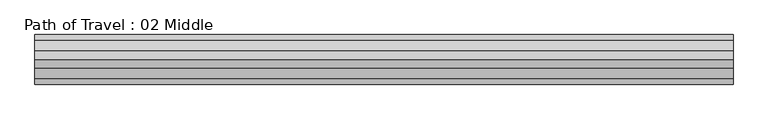
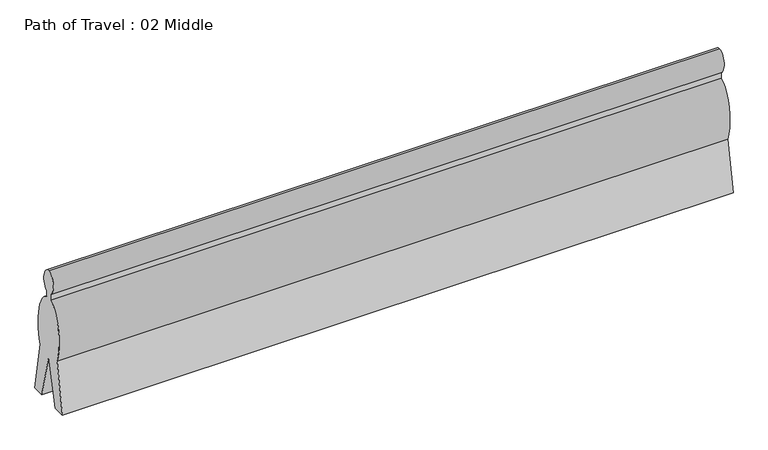
"""IFC4 building model written with IfcOpenShell, lengths in millimetres: proxy geometry, Path of Travel : 02 Middle."""

from ifc_helpers import new_model, si_unit, point, frame, origin, place, context, project, spatial, ellipse_curve, trimmed, source, transform, mapped, element, save
from ifc_brep_helpers import plane_surface, extruded_surface, advanced_brep


def path_of_travel_02_middle_f5177a39(model_context):
    return source(origin(), model_context, "Body", "AdvancedBrep", [
        advanced_brep(
        [(227.5554837, 0.0, 1727.2), (227.5554837, 42.9018657, 1436.6534209), (227.5554837, 42.9018657, 1363.4763406), (227.5554837, 184.1186263, 643.4144547), (227.5554837, 297.5699544, 0.0), (227.5554837, 145.6574193, 0.0), (227.5554837, 0.0, 584.2), (227.5554837, -145.6574193, 0.0), (227.5554837, -297.5699544, 0.0), (227.5554837, -184.1186263, 643.4144547), (227.5554837, -42.9018657, 1363.4763406), (227.5554837, -42.9018657, 1436.6534209), (8609.5554837, 0.0, 1727.2), (8609.5554837, -42.9018657, 1436.6534209), (8609.5554837, -42.9018657, 1363.4763406), (8609.5554837, -184.1186263, 643.4144547), (8609.5554837, -297.5699544, 0.0), (8609.5554837, -145.6574193, 0.0), (8609.5554837, 0.0, 584.2), (8609.5554837, 145.6574193, 0.0), (8609.5554837, 297.5699544, 0.0), (8609.5554837, 184.1186263, 643.4144547), (8609.5554837, 42.9018657, 1363.4763406), (8609.5554837, 42.9018657, 1436.6534209)],
        [
            (0, 1, ellipse_curve(frame((227.5554837, 0.0, 1574.8), z_axis=(-1.0, 0.0, 0.0), x_axis=(0.0, 0.0, 1.0)), 152.4, 101.6)),
            (1, 2),
            (2, 3, ellipse_curve(frame((227.5554837, 0.0, 914.4), z_axis=(-1.0, 0.0, 0.0), x_axis=(0.0, 0.0, -1.0)), 457.2, 228.6)),
            (3, 4),
            (4, 5),
            (5, 6),
            (6, 7),
            (7, 8),
            (8, 9),
            (9, 10, ellipse_curve(frame((227.5554837, 0.0, 914.4), z_axis=(-1.0, 0.0, 0.0), x_axis=(0.0, 0.0, -1.0)), 457.2, 228.6)),
            (10, 11),
            (11, 0, ellipse_curve(frame((227.5554837, 0.0, 1574.8), z_axis=(-1.0, 0.0, 0.0), x_axis=(0.0, 0.0, 1.0)), 152.4, 101.6)),
            (12, 13, ellipse_curve(frame((8609.5554837, 0.0, 1574.8), z_axis=(1.0, 0.0, 0.0), x_axis=(0.0, 0.0, 1.0)), 152.4, 101.6)),
            (13, 14),
            (14, 15, ellipse_curve(frame((8609.5554837, 0.0, 914.4), z_axis=(1.0, 0.0, 0.0), x_axis=(0.0, 0.0, -1.0)), 457.2, 228.6)),
            (15, 16),
            (16, 17),
            (17, 18),
            (18, 19),
            (19, 20),
            (20, 21),
            (21, 22, ellipse_curve(frame((8609.5554837, 0.0, 914.4), z_axis=(1.0, 0.0, 0.0), x_axis=(0.0, 0.0, -1.0)), 457.2, 228.6)),
            (22, 23),
            (23, 12, ellipse_curve(frame((8609.5554837, 0.0, 1574.8), z_axis=(1.0, 0.0, 0.0), x_axis=(0.0, 0.0, 1.0)), 152.4, 101.6)),
            (0, 12),
            (23, 1),
            (22, 2),
            (21, 3),
            (20, 4),
            (19, 5),
            (18, 6),
            (17, 7),
            (16, 8),
            (15, 9),
            (14, 10),
            (13, 11),
        ],
        [
            plane_surface(frame((227.5554837, 0.0, 0.0), z_axis=(-1.0, 0.0, 0.0), x_axis=(0.0, 0.0, 1.0))),
            plane_surface(frame((8609.5554837, 0.0, 0.0), z_axis=(1.0, 0.0, 0.0), x_axis=(0.0, 0.0, 1.0))),
            extruded_surface(trimmed(ellipse_curve(frame((8609.5554837, 0.0, 1574.8), z_axis=(-1.0, 0.0, 0.0), x_axis=(0.0, 0.0, 1.0)), 152.4, 101.6), [point((8609.5554837, 0.0, 1727.2))], [point((8609.5554837, 42.9018657, 1436.6534209))], True, "CARTESIAN"), (-8382.0, 0.0, 0.0), 8382.0),
            plane_surface(frame((227.5554837, 42.9018657, 1436.6534209), z_axis=(0.0, 1.0, 0.0), x_axis=(1.0, 0.0, 0.0))),
            extruded_surface(trimmed(ellipse_curve(frame((8609.5554837, 0.0, 914.4), z_axis=(-1.0, 0.0, 0.0), x_axis=(0.0, 0.0, -1.0)), 457.2, 228.6), [point((8609.5554837, 42.9018657, 1363.4763406))], [point((8609.5554837, 184.1186263, 643.4144547))], True, "CARTESIAN"), (-8382.0, 0.0, 0.0), 8382.0),
            plane_surface(frame((227.5554837, 184.1186263, 643.4144547), z_axis=(0.0, 0.9848077530122078, 0.17364817766693205), x_axis=(1.0, 0.0, 0.0))),
            plane_surface(frame((227.5554837, 297.5699544, 0.0), z_axis=(0.0, 0.0, -1.0), x_axis=(1.0, 0.0, 0.0))),
            plane_surface(frame((227.5554837, 145.6574193, 0.0), z_axis=(0.0, -0.9702957262760199, -0.2419218955995739), x_axis=(1.0, 0.0, 0.0))),
            plane_surface(frame((227.5554837, 0.0, 584.2), z_axis=(0.0, 0.9702957262759961, -0.24192189559966923), x_axis=(1.0, 0.0, 0.0))),
            plane_surface(frame((227.5554837, -145.6574193, 0.0), z_axis=(0.0, 0.0, -1.0), x_axis=(1.0, 0.0, 0.0))),
            plane_surface(frame((227.5554837, -297.5699544, 0.0), z_axis=(0.0, -0.984807753012208, 0.17364817766693066), x_axis=(1.0, 0.0, 0.0))),
            extruded_surface(trimmed(ellipse_curve(frame((8609.5554837, 0.0, 914.4), z_axis=(-1.0, 0.0, 0.0), x_axis=(0.0, 0.0, -1.0)), 457.2, 228.6), [point((8609.5554837, -184.1186263, 643.4144547))], [point((8609.5554837, -42.9018657, 1363.4763406))], True, "CARTESIAN"), (-8382.0, 0.0, 0.0), 8382.0),
            plane_surface(frame((227.5554837, -42.9018657, 1363.4763406), z_axis=(0.0, -1.0, 0.0), x_axis=(1.0, 0.0, 0.0))),
            extruded_surface(trimmed(ellipse_curve(frame((8609.5554837, 0.0, 1574.8), z_axis=(-1.0, 0.0, 0.0), x_axis=(0.0, 0.0, 1.0)), 152.4, 101.6), [point((8609.5554837, -42.9018657, 1436.6534209))], [point((8609.5554837, 0.0, 1727.2))], True, "CARTESIAN"), (-8382.0, 0.0, 0.0), 8382.0),
        ],
        [
            (0, [[1, 2, 3, 4, 5, 6, 7, 8, 9, 10, 11, 12]]),
            (1, [[13, 14, 15, 16, 17, 18, 19, 20, 21, 22, 23, 24]]),
            (2, [[-1, 25, -24, 26]]),
            (3, [[-2, -26, -23, 27]]),
            (4, [[-3, -27, -22, 28]]),
            (5, [[-4, -28, -21, 29]]),
            (6, [[-5, -29, -20, 30]]),
            (7, [[-6, -30, -19, 31]]),
            (8, [[-7, -31, -18, 32]]),
            (9, [[-8, -32, -17, 33]]),
            (10, [[-9, -33, -16, 34]]),
            (11, [[-10, -34, -15, 35]]),
            (12, [[-11, -35, -14, 36]]),
            (13, [[-12, -36, -13, -25]]),
        ],
    ),
    ])


if __name__ == "__main__":
    model = new_model("IFC4")
    model_context = context("Model", 3, world=origin())
    ifc_project = project(units=[si_unit("LENGTHUNIT", "METRE", prefix="MILLI")], contexts=[model_context])
    site = spatial("IfcSite", under=ifc_project)
    building = spatial("IfcBuilding", under=site)
    placement = place(None, origin())
    path_of_travel_02_middle_shape = path_of_travel_02_middle_f5177a39(model_context)
    element("IfcBuildingElementProxy", 1, Name="Path of Travel : 02 Middle", ObjectType="Path of Travel : 02 Middle", at=placement, inside=building, context=model_context, shape_type="MappedRepresentation", body=[
        mapped(path_of_travel_02_middle_shape, transform((0.0, 0.0, 0.0), x_axis=(1.0, 0.0, 0.0), y_axis=(0.0, 1.0, 0.0), z_axis=(0.0, 0.0, 1.0))),
    ])
    save(model, "model.ifc")

# Revit data of these elements
# Type "Path of Travel : 02 Middle"
#   Path of Egress [instance default] = 4' - 0"
#   built-in parameter 1001306 [instance default] = 4 (stored number, unit not read)
#   Dot at Start = no
#   Arrow in Middle = yes
#   Arrow at End = no
#   Egress Path = none
# Element 1 (IfcBuildingElementProxy, "Path of Travel : 02 Middle")
#   Path of Egress = 27' - 6"
#   built-in parameter 1001306 = 27.5 (stored number, unit not read)
#   Materials on its faces: "Egress Path Solid"
# Materials
#   "Egress Path Solid": class "Unassigned", colour RGB 255 128 64, transparency 0.75, Comments = "Rendering appearance not upgraded "
